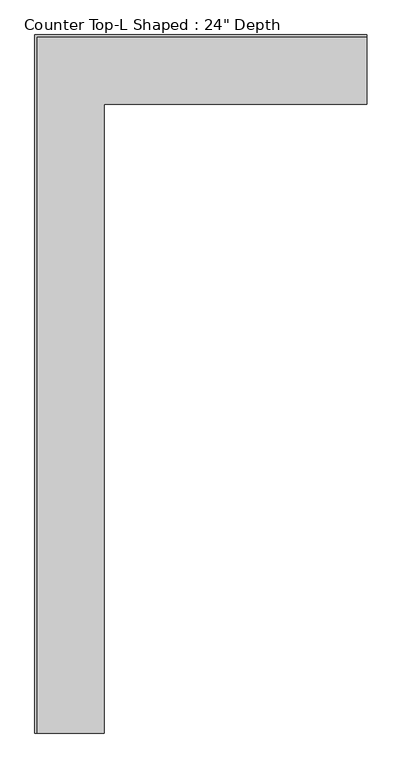
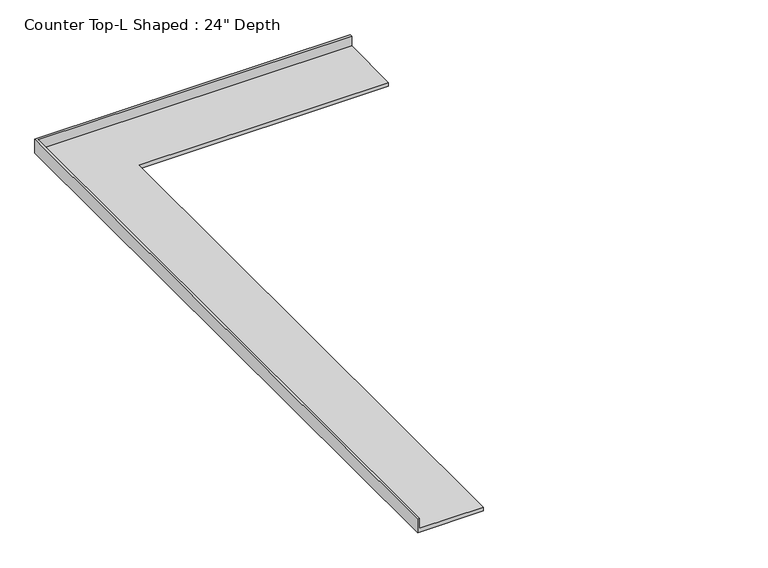
"""IFC4 building model written with IfcOpenShell, lengths in millimetres: furniture geometry."""

from ifc_helpers import new_model, si_unit, origin, place, context, project, spatial, faceted_brep, source, transform, mapped, element, save


def furniture_941a21fa(model_context):
    return source(origin(), model_context, "Body", "Brep", [
        faceted_brep([(-565.4622951, -6400.8, 914.4), (-565.4622951, -635.0, 914.4), (1847.5377049, -635.0, 914.4), (1847.5377049, -19.05, 914.4), (-1181.4122951, -19.05, 914.4), (-1181.4122951, -6400.8, 914.4), (1847.5377049, 0.0, 876.3), (1847.5377049, -635.0, 876.3), (-565.4622951, -635.0, 876.3), (-565.4622951, -6400.8, 876.3), (-1200.4622951, -6400.8, 876.3), (-1200.4622951, 0.0, 876.3), (-1200.4622951, 0.0, 1016.0), (1847.5377049, 0.0, 1016.0), (-1200.4622951, -6400.8, 1016.0), (-1181.4122951, -6400.8, 1016.0), (1847.5377049, -19.05, 1016.0), (-1181.4122951, -19.05, 1016.0)], [[[0, 1, 2, 3, 4, 5]], [[6, 7, 8, 9, 10, 11]], [[6, 11, 12, 13]], [[11, 10, 14, 12]], [[14, 10, 9, 0, 5, 15]], [[1, 0, 9, 8]], [[2, 1, 8, 7]], [[7, 6, 13, 16, 3, 2]], [[12, 14, 15, 17, 16, 13]], [[3, 16, 17, 4]], [[17, 15, 5, 4]]]),
    ])


if __name__ == "__main__":
    model = new_model("IFC4")
    model_context = context("Model", 3, world=origin())
    ifc_project = project(units=[si_unit("LENGTHUNIT", "METRE", prefix="MILLI")], contexts=[model_context])
    site = spatial("IfcSite", under=ifc_project)
    building = spatial("IfcBuilding", under=site)
    placement = place(None, origin())
    furniture_shape = furniture_941a21fa(model_context)
    element("IfcFurniture", 1, ObjectType="Counter Top-L Shaped : 24\" Depth", at=placement, inside=building, context=model_context, shape_type="MappedRepresentation", body=[
        mapped(furniture_shape, transform((0.0, 0.0, 0.0), x_axis=(1.0, 0.0, 0.0), y_axis=(0.0, 1.0, 0.0), z_axis=(0.0, 0.0, 1.0))),
    ])
    save(model, "model.ifc")

# Revit data of these elements
# Type "Counter Top-L Shaped : 24\" Depth"
#   Assembly Code = "C1030400"
#   Counter Thickness = 0' - 1 1/2"
#   Depth = 2' - 1"
#   Height = 3' - 0"
#   Length - Leg 1 [instance default] = 8' - 0"
#   Length - Leg 2 [instance default] = 6' - 0"
#   Counter Top Material = none
#   Default Elevation = 0
# Element 1 (IfcFurniture, "Counter Top-L Shaped : 24\" Depth")
#   Length - Leg 1 = 10' - 0"
#   Length - Leg 2 = 21' - 0"
#   Materials on its faces: "Counter Top"
# Materials
#   "Counter Top": class "Wood", colour RGB 226 177 128, transparency 0, Cost = 0
